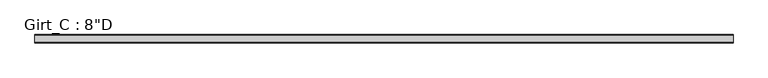
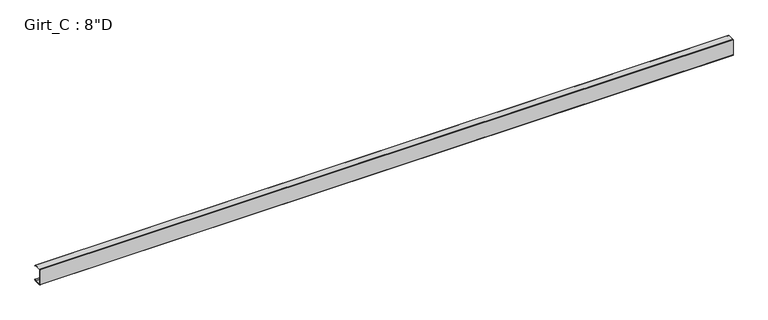
"""IFC4 building model written with IfcOpenShell, lengths in millimetres: beam geometry."""

from ifc_helpers import new_model, si_unit, point, frame, frame_2d, origin, place, context, project, spatial, polyline, circle_curve, trimmed, segment, composite_curve, outline, extrude, source, transform, mapped, element, save


def beam_2282d545(model_context):
    return source(origin(), model_context, "Body", "SweptSolid", [
        extrude(outline(composite_curve([segment(polyline([(87.5109375, 101.6), (99.7560415, 87.0068534), (97.6278742, 85.221109), (86.2154765, 98.821875), (3.3005807, 98.821875)]), True, "CONTINUOUS"), segment(trimmed(circle_curve(frame_2d((3.3741066, 96.8381931)), 1.9850441), [point((3.3005807, 98.821875))], [point((1.3890625, 96.8381931))], True, "CARTESIAN"), True, "CONTINUOUS"), segment(polyline([(1.3890625, 96.8381931), (1.3890625, -96.8389339)]), True, "CONTINUOUS"), segment(trimmed(circle_curve(frame_2d((3.3748024, -96.8389339)), 1.9857399), [point((1.3890625, -96.8389339))], [point((3.2694106, -98.821875))], True, "CARTESIAN"), True, "CONTINUOUS"), segment(polyline([(3.2694106, -98.821875), (86.2154765, -98.821875), (97.6510975, -85.1934327), (99.7792647, -86.979177), (87.5109375, -101.6), (3.3734375, -101.6)]), True, "CONTINUOUS"), segment(trimmed(circle_curve(frame_2d((3.3734375, -96.8375)), 4.7625), [point((3.3734375, -101.6))], [point((-1.3890625, -96.8375))], False, "CARTESIAN"), True, "CONTINUOUS"), segment(polyline([(-1.3890625, -96.8375), (-1.3890625, 96.8375)]), True, "CONTINUOUS"), segment(trimmed(circle_curve(frame_2d((3.3734375, 96.8375)), 4.7625), [point((-1.3890625, 96.8375))], [point((3.3734375, 101.6))], False, "CARTESIAN"), True, "CONTINUOUS"), segment(polyline([(3.3734375, 101.6), (87.5109375, 101.6)]), True, "CONTINUOUS")], self_intersect=False)), frame((-4348.559375, 0.0, 0.0), z_axis=(1.0, 0.0, 0.0), x_axis=(0.0, 1.0, 0.0)), (0.0, 0.0, 1.0), 8531.225),
    ])


if __name__ == "__main__":
    model = new_model("IFC4")
    model_context = context("Model", 3, world=origin())
    ifc_project = project(units=[si_unit("LENGTHUNIT", "METRE", prefix="MILLI")], contexts=[model_context])
    site = spatial("IfcSite", under=ifc_project)
    building = spatial("IfcBuilding", under=site)
    placement = place(None, origin())
    beam_shape = beam_2282d545(model_context)
    element("IfcBeam", 1, ObjectType="Girt_C : 8\"D", at=placement, inside=building, context=model_context, shape_type="MappedRepresentation", body=[
        mapped(beam_shape, transform((0.0, 0.0, 0.0), x_axis=(1.0, 0.0, 0.0), y_axis=(0.0, 1.0, 0.0), z_axis=(0.0, 0.0, 1.0))),
    ])
    save(model, "model.ifc")

# Revit data of these elements
# Project information
#   Project Issue Date = "07/20/2015"
#   Project Status = "Project Status"
#   Client Name = "Xcel"
#   Project Address = "Enter address here"
#   Project Name = "Xcel Sports Complex"
#   Project Number = "Project Number"
# Type "Girt_C : 8\"D"
#   half leg = 0' - 1 3/4"
#   Web_Thickness = 0' - 0 7/64"
#   Length [instance default] = 10' - 0"
#   Leg_1 = 0' - 3 1/2"
#   Height = 0' - 8"
#   Structural Material [instance default] = none
# Element 1 (IfcBeam, "Girt_C : 8\"D")
#   Structural Material = GALVANIZED 'CEE' SECTION (8.0x3.5C - SEE STRUCT. DWGS)
#   Materials on its faces: "GALVANIZED 'CEE' SECTION (8.0x3.5C - SEE STRUCT. DWGS)"
# Materials
#   "GALVANIZED 'CEE' SECTION (8.0x3.5C - SEE STRUCT. DWGS)": class "Metal", colour RGB 137 146 153, transparency 0, Description = "Steel, mill finish", Cost = 0
